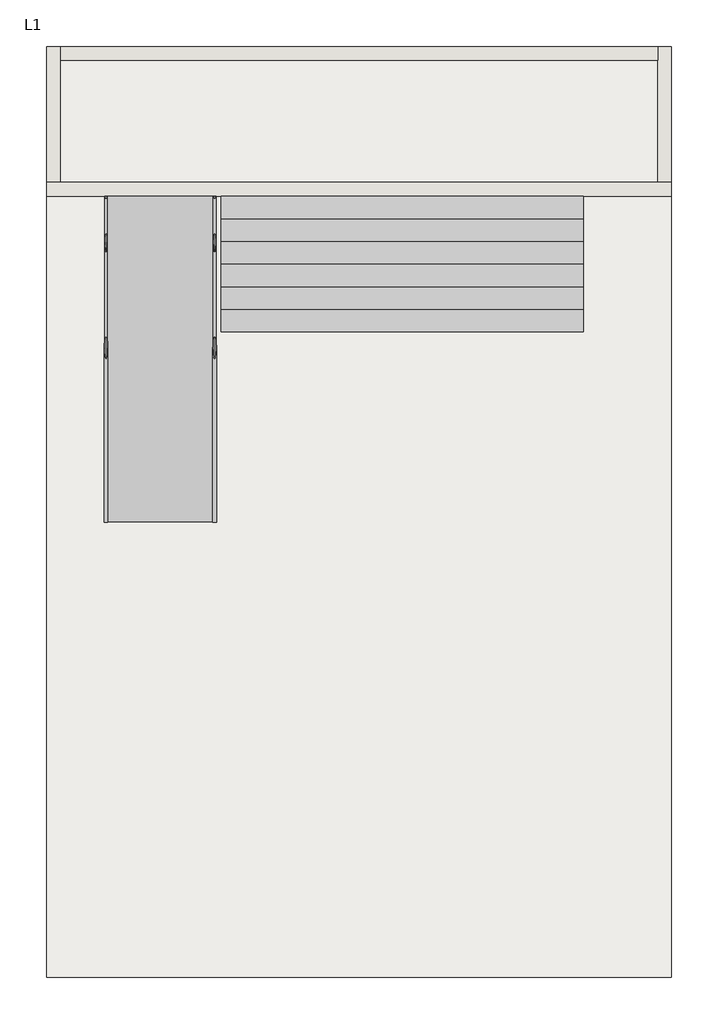
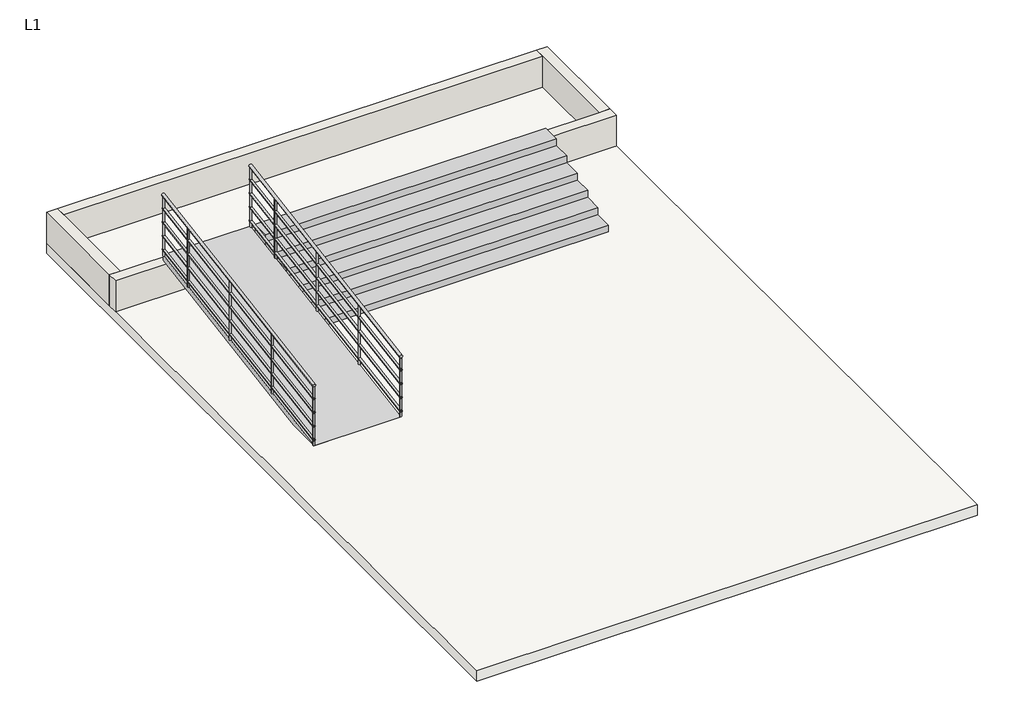
# One storey: 4 walls, 2 railings, 1 ramp, 1 slab, 1 stair flight.
"""IFC4 building model written with IfcOpenShell, lengths in millimetres."""

import ifcopenshell
import ifcopenshell.guid

model = None  # the IFC model being written
_history = None  # IfcOwnerHistory: only IFC2X3 demands one
_inside = {}  # id of a spatial element -> (the spatial element, [elements in it])
_under = {}  # id of a project, library or spatial element -> (it, [spatial elements below it])
_declared = {}  # id of a project -> (the project, [libraries it declares])
_typed = {}  # id of a type object -> (the type object, [elements of that type])
_made_of = {}  # id of a material, layer set ... -> (it, [elements and type objects made of it])


def new_model(schema):
    """Start an empty IFC model of exactly this schema.

    Asked for "IFC4X3", IfcOpenShell would pick the latest addendum, in which some entities
    have other attributes; the version numbers below select the first issue.
    IFC2X3 requires an IfcOwnerHistory on every rooted entity: one is made here for all.
    """
    global model, _history
    if schema == "IFC4X3":
        model = ifcopenshell.file(schema_version=(4, 3, 0, 0))
    else:
        model = ifcopenshell.file(schema=schema)
    _inside.clear()
    _under.clear()
    _declared.clear()
    _typed.clear()
    _made_of.clear()
    _history = None
    if model.schema == "IFC2X3":
        org = make("IfcOrganization", Name="unknown")
        user = make(
            "IfcPersonAndOrganization",
            ThePerson=make("IfcPerson", FamilyName="unknown"),
            TheOrganization=org,
        )
        app = make(
            "IfcApplication",
            ApplicationDeveloper=org,
            Version="unknown",
            ApplicationFullName="unknown",
            ApplicationIdentifier="unknown",
        )
        _history = make(
            "IfcOwnerHistory",
            OwningUser=user,
            OwningApplication=app,
            ChangeAction="ADDED",
            CreationDate=0,
        )
    return model


def make(cls, **values):
    """One entity of the class cls with the attributes given. An attribute that is None is left unset."""
    return model.create_entity(
        cls, **{name: value for name, value in values.items() if value is not None}
    )


def rooted(cls, **values):
    """An entity with a GlobalId (a new one), such as an element, a storey or a relation."""
    return make(cls, GlobalId=ifcopenshell.guid.new(), OwnerHistory=_history, **values)


def si_unit(unit_type, name, prefix=None):
    """IfcSIUnit, for example si_unit("LENGTHUNIT", "METRE", prefix="MILLI")."""
    return make("IfcSIUnit", UnitType=unit_type, Prefix=prefix, Name=name)


def assignment(units):
    """IfcUnitAssignment: the units of a project."""
    return None if units is None else make("IfcUnitAssignment", Units=units)


def point(xyz):
    """IfcCartesianPoint."""
    return None if xyz is None else make("IfcCartesianPoint", Coordinates=xyz)


def direction(xyz):
    """IfcDirection."""
    return None if xyz is None else make("IfcDirection", DirectionRatios=xyz)


def frame(location, z_axis=None, x_axis=None):
    """IfcAxis2Placement3D, a coordinate frame: its origin and axes. An axis left out is left unset."""
    return make(
        "IfcAxis2Placement3D",
        Location=point(location),
        Axis=direction(z_axis),
        RefDirection=direction(x_axis),
    )


def origin():
    """The frame at (0, 0, 0) with its axes left unset."""
    return frame((0.0, 0.0, 0.0))


def origin_with_axes():
    """The frame at (0, 0, 0) with the z axis (0, 0, 1) and the x axis (1, 0, 0) written out."""
    return frame((0.0, 0.0, 0.0), z_axis=(0.0, 0.0, 1.0), x_axis=(1.0, 0.0, 0.0))


def place(relative_to, where):
    """IfcLocalPlacement: puts the frame where relative to a parent placement (None: the world)."""
    return make(
        "IfcLocalPlacement", PlacementRelTo=relative_to, RelativePlacement=where
    )


def context(
    kind, dimensions, precision=None, world=None, true_north=None, identifier=None
):
    """IfcGeometricRepresentationContext, for example the 3D "Model" context."""
    return make(
        "IfcGeometricRepresentationContext",
        ContextIdentifier=identifier,
        ContextType=kind,
        CoordinateSpaceDimension=dimensions,
        Precision=precision,
        WorldCoordinateSystem=world,
        TrueNorth=true_north,
    )


def project(units=None, contexts=None):
    """IfcProject with its units and contexts."""
    return rooted(
        "IfcProject",
        Name="project",
        RepresentationContexts=contexts,
        UnitsInContext=assignment(units),
    )


def spatial(cls, under=None, at=None, **own):
    """A site, building, storey or space (cls), placed at a placement, below another one or the project."""
    s = rooted(cls, ObjectPlacement=at, **own)
    if under is not None:
        _under.setdefault(under.id(), (under, []))[1].append(s)
    return s


def polyline(points):
    """IfcPolyline through the points."""
    return make("IfcPolyline", Points=[point(p) for p in points])


def ellipse_curve(where, semi_axis1, semi_axis2):
    """IfcEllipse in the frame where."""
    return make(
        "IfcEllipse", Position=where, SemiAxis1=semi_axis1, SemiAxis2=semi_axis2
    )


def outline(outer, holes=None, kind="AREA"):
    """IfcArbitraryClosedProfileDef: a profile drawn as a closed curve; with holes, ...WithVoids."""
    if holes is None:
        return make("IfcArbitraryClosedProfileDef", ProfileType=kind, OuterCurve=outer)
    return make(
        "IfcArbitraryProfileDefWithVoids",
        ProfileType=kind,
        OuterCurve=outer,
        InnerCurves=holes,
    )


def extrude(swept, where, along, depth):
    """IfcExtrudedAreaSolid: the profile swept, set in the frame where, extruded along a direction by depth."""
    return make(
        "IfcExtrudedAreaSolid",
        SweptArea=swept,
        Position=where,
        ExtrudedDirection=direction(along),
        Depth=depth,
    )


def faces_of(points, faces, orient=None, outer=None):
    """IfcFace entities. A face is a list of loops; a loop is a list of indices into points, from 0.

    orient and outer hold one flag for each loop. By default every Orientation is true, the
    first loop of a face is its IfcFaceOuterBound and the others are IfcFaceBound.
    """
    made = []
    for i, loops in enumerate(faces):
        bounds = []
        for j, loop in enumerate(loops):
            is_outer = j == 0 if outer is None else outer[i][j]
            bounds.append(
                make(
                    "IfcFaceOuterBound" if is_outer else "IfcFaceBound",
                    Bound=make("IfcPolyLoop", Polygon=[points[k] for k in loop]),
                    Orientation=True if orient is None else orient[i][j],
                )
            )
        made.append(make("IfcFace", Bounds=bounds))
    return made


def faceted_brep(points, faces, orient=None, outer=None, voids=None):
    """IfcFacetedBrep: a solid bounded by flat faces; with voids (closed shells), ...WithVoids."""
    shared = [point(p) for p in points]
    hull = make("IfcClosedShell", CfsFaces=faces_of(shared, faces, orient, outer))
    if voids is None:
        return make("IfcFacetedBrep", Outer=hull)
    return make(
        "IfcFacetedBrepWithVoids",
        Outer=hull,
        Voids=[
            make(cls, CfsFaces=faces_of(shared, fs, o, b)) for cls, fs, o, b in voids
        ],
    )


def shape(context_of_items, identifier, shape_type, items):
    """IfcShapeRepresentation: the items that make up one representation, for example the "Body"."""
    return make(
        "IfcShapeRepresentation",
        ContextOfItems=context_of_items,
        RepresentationIdentifier=identifier,
        RepresentationType=shape_type,
        Items=items,
    )


def source(mapping_origin, context_of_items, identifier, shape_type, items):
    """IfcRepresentationMap: a shape defined once, which mapped items show again and again."""
    return make(
        "IfcRepresentationMap",
        MappingOrigin=mapping_origin,
        MappedRepresentation=shape(context_of_items, identifier, shape_type, items),
    )


def transform(
    local_origin,
    x_axis=None,
    y_axis=None,
    z_axis=None,
    scale=None,
    scale2=None,
    scale3=None,
    uniform=True,
):
    """IfcCartesianTransformationOperator3D, or its non-uniform kind. x_axis, y_axis, z_axis: its Axis1, 2, 3."""
    if uniform:
        return make(
            "IfcCartesianTransformationOperator3D",
            Axis1=direction(x_axis),
            Axis2=direction(y_axis),
            LocalOrigin=point(local_origin),
            Scale=scale,
            Axis3=direction(z_axis),
        )
    return make(
        "IfcCartesianTransformationOperator3DnonUniform",
        Axis1=direction(x_axis),
        Axis2=direction(y_axis),
        LocalOrigin=point(local_origin),
        Scale=scale,
        Axis3=direction(z_axis),
        Scale2=scale2,
        Scale3=scale3,
    )


def mapped(mapping_source, mapping_target):
    """IfcMappedItem: shows the shape of a source again, moved by a transform."""
    return make(
        "IfcMappedItem", MappingSource=mapping_source, MappingTarget=mapping_target
    )


def made_of(thing, what):
    """Note that an element or type object is made of a material, layer set ...; save() writes the relation."""
    if what is not None:
        _made_of.setdefault(what.id(), (what, []))[1].append(thing)
    return thing


def element(
    cls,
    number,
    at=None,
    inside=None,
    cuts=None,
    type_object=None,
    material=None,
    context=None,
    identifier="Body",
    shape_type=None,
    held_by="IfcProductDefinitionShape",
    body=None,
    shapes=None,
    **own,
):
    """One element of the class cls, such as IfcWall. Its Tag is "e" and its number.

    at: its placement. inside: the storey or other place that contains it. cuts: it is an
    opening in that element (IfcRelVoidsElement). A single representation is given by context,
    identifier, shape_type and body (its items); several are given by shapes. held_by: the class
    of the entity that holds the representations. save() writes the other relations.
    """
    e = rooted(cls, Tag="e%d" % number, ObjectPlacement=at, **own)
    if body is not None:
        shapes = [shape(context, identifier, shape_type, body)]
    if shapes is not None:
        e.Representation = make(held_by, Representations=shapes)
    if inside is not None:
        _inside.setdefault(inside.id(), (inside, []))[1].append(e)
    if cuts is not None:
        rooted(
            "IfcRelVoidsElement", RelatingBuildingElement=cuts, RelatedOpeningElement=e
        )
    if type_object is not None:
        _typed.setdefault(type_object.id(), (type_object, []))[1].append(e)
    return made_of(e, material)


def aggregate(whole, parts):
    """IfcRelAggregates: a whole, such as a stair, and the parts it consists of."""
    return rooted("IfcRelAggregates", RelatingObject=whole, RelatedObjects=parts)


def save(model, path):
    """Write the relations noted so far, then the file.

    IfcRelAggregates (storeys below a building ...), IfcRelContainedInSpatialStructure (elements
    in a storey), IfcRelDefinesByType, IfcRelAssociatesMaterial and IfcRelDeclares: one each for
    every whole, place, type object, material and project.
    """
    for whole, parts in _under.values():
        aggregate(whole, parts)
    for where, things in _inside.values():
        rooted(
            "IfcRelContainedInSpatialStructure",
            RelatedElements=things,
            RelatingStructure=where,
        )
    for kind, things in _typed.values():
        rooted("IfcRelDefinesByType", RelatedObjects=things, RelatingType=kind)
    for what, things in _made_of.values():
        rooted("IfcRelAssociatesMaterial", RelatedObjects=things, RelatingMaterial=what)
    for by, libraries in _declared.values():
        rooted("IfcRelDeclares", RelatingContext=by, RelatedDefinitions=libraries)
    model.write(path)


def plane_surface(at):
    """IfcPlane: the flat surface through the origin of the frame at, square to its z axis."""
    return make("IfcPlane", Position=at)


def cylinder_surface(at, radius):
    """IfcCylindricalSurface: all points at the distance radius from the z axis of the frame at."""
    return make("IfcCylindricalSurface", Position=at, Radius=radius)


def advanced_brep(points, edges, surfaces, faces):
    """IfcAdvancedBrep: a solid bounded by faces that lie on surfaces and meet in shared edges.

    An edge is (start, end): straight between two places in points (the first is 0);
    or (start, end, curve); or (start, end, curve, False) where it runs against its curve.
    A face is (place in surfaces, loops), or (place, loops, False) where it looks against
    its surface's normal. A loop lists edges by number (the first is 1), with a minus sign
    where the edge is run from its end to its start. The first loop is the outer one.
    """
    corners = [point(p) for p in points]
    vertices = [make("IfcVertexPoint", VertexGeometry=c) for c in corners]
    made = []
    for start, end, *more in edges:
        made.append(
            make(
                "IfcEdgeCurve",
                EdgeStart=vertices[start],
                EdgeEnd=vertices[end],
                EdgeGeometry=more[0] if more else make("IfcPolyline", Points=[corners[start], corners[end]]),
                SameSense=more[1] if len(more) > 1 else True,
            )
        )
    hull = []
    for where, loops, *sense in faces:
        bounds = []
        for j, loop in enumerate(loops):
            ring = [make("IfcOrientedEdge", EdgeElement=made[abs(k) - 1], Orientation=k > 0) for k in loop]
            bounds.append(
                make(
                    "IfcFaceOuterBound" if j == 0 else "IfcFaceBound",
                    Bound=make("IfcEdgeLoop", EdgeList=ring),
                    Orientation=True,
                )
            )
        hull.append(make("IfcAdvancedFace", Bounds=bounds, FaceSurface=surfaces[where], SameSense=sense[0] if sense else True))
    return make("IfcAdvancedBrep", Outer=make("IfcClosedShell", CfsFaces=hull))


def ramp_1_7f35b39e(model_context):
    return source(origin(), model_context, "Body", "SweptSolid", [
        extrude(outline(polyline([(-4458.4292912, 0.0), (-858.4292912, 600.0), (-858.4292912, 523.9654684), (-4458.4292912, -76.0345316), (-4458.4292912, 0.0)])), frame((-599.8488078, 0.0, 0.0), z_axis=(1.0, 0.0, 0.0), x_axis=(0.0, 1.0, 0.0)), (0.0, 0.0, 1.0), 1200.0),
    ])


model = new_model("IFC4")

# Units and contexts
model_context = context("Model", 3, world=origin())
ifc_project = project(units=[si_unit("LENGTHUNIT", "METRE", prefix="MILLI")], contexts=[model_context])

# Site, building, storey
site = spatial("IfcSite", under=ifc_project)
building = spatial("IfcBuilding", under=site)
storey = spatial("IfcBuildingStorey", under=building, Name="L1", Elevation=0.0)

# Railings
placement = place(None, origin())
element("IfcRailing", 1, ObjectType="900mm Pipe", at=placement, inside=storey, context=model_context, shape_type="AdvancedBrep", body=[
    advanced_brep(
    [(620.1511922, -4458.4292912, 879.7241249), (580.1511922, -4458.4292912, 879.7241249), (620.1511922, -858.4292912, 1479.7241249), (580.1511922, -858.4292912, 1479.7241249)],
    [
        (0, 1, ellipse_curve(frame((600.1511922, -4458.4292912, 879.7241249), z_axis=(0.0, -1.0, 0.0), x_axis=(0.0, 0.0, -1.0)), 20.2758751, 20.0)),
        (1, 0, ellipse_curve(frame((600.1511922, -4458.4292912, 879.7241249), z_axis=(0.0, -1.0, 0.0), x_axis=(0.0, 0.0, -1.0)), 20.2758751, 20.0)),
        (2, 3, ellipse_curve(frame((600.1511922, -858.4292912, 1479.7241249), z_axis=(0.0, 1.0, 0.0), x_axis=(0.0, 0.0, -1.0)), 20.2758751, 20.0)),
        (3, 2, ellipse_curve(frame((600.1511922, -858.4292912, 1479.7241249), z_axis=(0.0, 1.0, 0.0), x_axis=(0.0, 0.0, -1.0)), 20.2758751, 20.0)),
        (0, 2),
        (3, 1),
    ],
    [
        plane_surface(frame((600.1511922, -4458.4292912, 900.0), z_axis=(0.0, -1.0, 0.0), x_axis=(0.0, 0.0, 1.0))),
        plane_surface(frame((600.1511922, -858.4292912, 1500.0), z_axis=(0.0, 1.0, 0.0), x_axis=(0.0, 0.0, 1.0))),
        cylinder_surface(frame((600.1511922, -4455.1413114, 880.2721215), z_axis=(0.0, -0.9863939238321437, -0.16439898730535737), x_axis=(-1.0, 0.0, 0.0)), 20.0),
    ],
    [
        (0, [[1, 2]]),
        (1, [[3, 4]]),
        (2, [[-1, 5, -4, 6]]),
        (2, [[-2, -6, -3, -5]]),
    ],
),
    advanced_brep(
    [(615.1511922, -4458.4292912, 684.7930937), (585.1511922, -4458.4292912, 684.7930937), (615.1511922, -858.4292912, 1284.7930937), (585.1511922, -858.4292912, 1284.7930937)],
    [
        (0, 1, ellipse_curve(frame((600.1511922, -4458.4292912, 684.7930937), z_axis=(0.0, -1.0, 0.0), x_axis=(0.0, 0.0, -1.0)), 15.2069063, 15.0)),
        (1, 0, ellipse_curve(frame((600.1511922, -4458.4292912, 684.7930937), z_axis=(0.0, -1.0, 0.0), x_axis=(0.0, 0.0, -1.0)), 15.2069063, 15.0)),
        (2, 3, ellipse_curve(frame((600.1511922, -858.4292912, 1284.7930937), z_axis=(0.0, 1.0, 0.0), x_axis=(0.0, 0.0, -1.0)), 15.2069063, 15.0)),
        (3, 2, ellipse_curve(frame((600.1511922, -858.4292912, 1284.7930937), z_axis=(0.0, 1.0, 0.0), x_axis=(0.0, 0.0, -1.0)), 15.2069063, 15.0)),
        (0, 2),
        (3, 1),
    ],
    [
        plane_surface(frame((600.1511922, -4458.4292912, 700.0), z_axis=(0.0, -1.0, 0.0), x_axis=(0.0, 0.0, 1.0))),
        plane_surface(frame((600.1511922, -858.4292912, 1300.0), z_axis=(0.0, 1.0, 0.0), x_axis=(0.0, 0.0, 1.0))),
        cylinder_surface(frame((600.1511922, -4455.9633063, 685.2040911), z_axis=(0.0, -0.9863939238321437, -0.16439898730535732), x_axis=(-1.0, 0.0, 0.0)), 15.0),
    ],
    [
        (0, [[1, 2]]),
        (1, [[3, 4]]),
        (2, [[-1, 5, -4, 6]]),
        (2, [[-2, -6, -3, -5]]),
    ],
),
    advanced_brep(
    [(615.1511922, -4458.4292912, 484.7930937), (585.1511922, -4458.4292912, 484.7930937), (615.1511922, -858.4292912, 1084.7930937), (585.1511922, -858.4292912, 1084.7930937)],
    [
        (0, 1, ellipse_curve(frame((600.1511922, -4458.4292912, 484.7930937), z_axis=(0.0, -1.0, 0.0), x_axis=(0.0, 0.0, -1.0)), 15.2069063, 15.0)),
        (1, 0, ellipse_curve(frame((600.1511922, -4458.4292912, 484.7930937), z_axis=(0.0, -1.0, 0.0), x_axis=(0.0, 0.0, -1.0)), 15.2069063, 15.0)),
        (2, 3, ellipse_curve(frame((600.1511922, -858.4292912, 1084.7930937), z_axis=(0.0, 1.0, 0.0), x_axis=(0.0, 0.0, -1.0)), 15.2069063, 15.0)),
        (3, 2, ellipse_curve(frame((600.1511922, -858.4292912, 1084.7930937), z_axis=(0.0, 1.0, 0.0), x_axis=(0.0, 0.0, -1.0)), 15.2069063, 15.0)),
        (0, 2),
        (3, 1),
    ],
    [
        plane_surface(frame((600.1511922, -4458.4292912, 500.0), z_axis=(0.0, -1.0, 0.0), x_axis=(0.0, 0.0, 1.0))),
        plane_surface(frame((600.1511922, -858.4292912, 1100.0), z_axis=(0.0, 1.0, 0.0), x_axis=(0.0, 0.0, 1.0))),
        cylinder_surface(frame((600.1511922, -4455.9633063, 485.2040911), z_axis=(0.0, -0.9863939238321437, -0.16439898730535732), x_axis=(-1.0, 0.0, 0.0)), 15.0),
    ],
    [
        (0, [[1, 2]]),
        (1, [[3, 4]]),
        (2, [[-1, 5, -4, 6]]),
        (2, [[-2, -6, -3, -5]]),
    ],
),
    advanced_brep(
    [(615.1511922, -4458.4292912, 284.7930937), (585.1511922, -4458.4292912, 284.7930937), (615.1511922, -858.4292912, 884.7930937), (585.1511922, -858.4292912, 884.7930937)],
    [
        (0, 1, ellipse_curve(frame((600.1511922, -4458.4292912, 284.7930937), z_axis=(0.0, -1.0, 0.0), x_axis=(0.0, 0.0, -1.0)), 15.2069063, 15.0)),
        (1, 0, ellipse_curve(frame((600.1511922, -4458.4292912, 284.7930937), z_axis=(0.0, -1.0, 0.0), x_axis=(0.0, 0.0, -1.0)), 15.2069063, 15.0)),
        (2, 3, ellipse_curve(frame((600.1511922, -858.4292912, 884.7930937), z_axis=(0.0, 1.0, 0.0), x_axis=(0.0, 0.0, -1.0)), 15.2069063, 15.0)),
        (3, 2, ellipse_curve(frame((600.1511922, -858.4292912, 884.7930937), z_axis=(0.0, 1.0, 0.0), x_axis=(0.0, 0.0, -1.0)), 15.2069063, 15.0)),
        (0, 2),
        (3, 1),
    ],
    [
        plane_surface(frame((600.1511922, -4458.4292912, 300.0), z_axis=(0.0, -1.0, 0.0), x_axis=(0.0, 0.0, 1.0))),
        plane_surface(frame((600.1511922, -858.4292912, 900.0), z_axis=(0.0, 1.0, 0.0), x_axis=(0.0, 0.0, 1.0))),
        cylinder_surface(frame((600.1511922, -4455.9633063, 285.2040911), z_axis=(0.0, -0.9863939238321437, -0.16439898730535732), x_axis=(-1.0, 0.0, 0.0)), 15.0),
    ],
    [
        (0, [[1, 2]]),
        (1, [[3, 4]]),
        (2, [[-1, 5, -4, 6]]),
        (2, [[-2, -6, -3, -5]]),
    ],
),
    advanced_brep(
    [(615.1511922, -4458.4292912, 84.7930937), (585.1511922, -4458.4292912, 84.7930937), (615.1511922, -858.4292912, 684.7930937), (585.1511922, -858.4292912, 684.7930937)],
    [
        (0, 1, ellipse_curve(frame((600.1511922, -4458.4292912, 84.7930937), z_axis=(0.0, -1.0, 0.0), x_axis=(0.0, 0.0, -1.0)), 15.2069063, 15.0)),
        (1, 0, ellipse_curve(frame((600.1511922, -4458.4292912, 84.7930937), z_axis=(0.0, -1.0, 0.0), x_axis=(0.0, 0.0, -1.0)), 15.2069063, 15.0)),
        (2, 3, ellipse_curve(frame((600.1511922, -858.4292912, 684.7930937), z_axis=(0.0, 1.0, 0.0), x_axis=(0.0, 0.0, -1.0)), 15.2069063, 15.0)),
        (3, 2, ellipse_curve(frame((600.1511922, -858.4292912, 684.7930937), z_axis=(0.0, 1.0, 0.0), x_axis=(0.0, 0.0, -1.0)), 15.2069063, 15.0)),
        (0, 2),
        (3, 1),
    ],
    [
        plane_surface(frame((600.1511922, -4458.4292912, 100.0), z_axis=(0.0, -1.0, 0.0), x_axis=(0.0, 0.0, 1.0))),
        plane_surface(frame((600.1511922, -858.4292912, 700.0), z_axis=(0.0, 1.0, 0.0), x_axis=(0.0, 0.0, 1.0))),
        cylinder_surface(frame((600.1511922, -4455.9633063, 85.2040911), z_axis=(0.0, -0.9863939238321437, -0.16439898730535732), x_axis=(-1.0, 0.0, 0.0)), 15.0),
    ],
    [
        (0, [[1, 2]]),
        (1, [[3, 4]]),
        (2, [[-1, 5, -4, 6]]),
        (2, [[-2, -6, -3, -5]]),
    ],
),
    advanced_brep(
    [(587.6511922, -1458.4292912, 1359.4482498), (612.6511922, -1458.4292912, 1359.4482498), (612.6511922, -1458.4292912, 500.0), (587.6511922, -1458.4292912, 500.0)],
    [
        (0, 1, ellipse_curve(frame((600.1511922, -1458.4292912, 1359.4482498), z_axis=(0.0, 0.1643989873053573, -0.9863939238321439), x_axis=(0.0, 0.9863939238321439, 0.1643989873053556)), 12.6724219, 12.5)),
        (1, 2),
        (2, 3, ellipse_curve(frame((600.1511922, -1458.4292912, 500.0), z_axis=(0.0, -0.16439898730535726, 0.9863939238321439), x_axis=(0.0, 0.9863939238321439, 0.16439898730535563)), 12.6724219, 12.5)),
        (3, 0),
        (3, 2, ellipse_curve(frame((600.1511922, -1458.4292912, 500.0), z_axis=(0.0, -0.16439898730535726, 0.9863939238321439), x_axis=(0.0, 0.9863939238321439, 0.16439898730535563)), 12.6724219, 12.5)),
        (1, 0, ellipse_curve(frame((600.1511922, -1458.4292912, 1359.4482498), z_axis=(0.0, 0.1643989873053573, -0.9863939238321439), x_axis=(0.0, 0.9863939238321439, 0.1643989873053556)), 12.6724219, 12.5)),
    ],
    [
        cylinder_surface(frame((600.1511922, -1458.4292912, 400.0), z_axis=(0.0, 0.0, 1.0), x_axis=(1.0, 0.0, 0.0)), 12.5),
        plane_surface(frame((625.1511922, -1433.4292912, 1363.6149165), z_axis=(0.0, -0.1643989873053573, 0.9863939238321439), x_axis=(-1.0, 0.0, 0.0))),
        plane_surface(frame((625.1511922, -1483.4292912, 495.8333333), z_axis=(0.0, 0.16439898730535726, -0.9863939238321439), x_axis=(-1.0, 0.0, 0.0))),
    ],
    [
        (0, [[1, 2, 3, 4]]),
        (0, [[5, -2, 6, -4]]),
        (1, [[-6, -1]]),
        (2, [[-5, -3]]),
    ],
),
    advanced_brep(
    [(587.6511922, -2458.4292912, 1192.7815831), (612.6511922, -2458.4292912, 1192.7815831), (612.6511922, -2458.4292912, 333.3333333), (587.6511922, -2458.4292912, 333.3333333)],
    [
        (0, 1, ellipse_curve(frame((600.1511922, -2458.4292912, 1192.7815831), z_axis=(0.0, 0.1643989873053573, -0.9863939238321439), x_axis=(0.0, 0.9863939238321439, 0.1643989873053556)), 12.6724219, 12.5)),
        (1, 2),
        (2, 3, ellipse_curve(frame((600.1511922, -2458.4292912, 333.3333333), z_axis=(0.0, -0.16439898730535726, 0.9863939238321439), x_axis=(0.0, 0.9863939238321439, 0.16439898730535563)), 12.6724219, 12.5)),
        (3, 0),
        (3, 2, ellipse_curve(frame((600.1511922, -2458.4292912, 333.3333333), z_axis=(0.0, -0.16439898730535726, 0.9863939238321439), x_axis=(0.0, 0.9863939238321439, 0.16439898730535563)), 12.6724219, 12.5)),
        (1, 0, ellipse_curve(frame((600.1511922, -2458.4292912, 1192.7815831), z_axis=(0.0, 0.1643989873053573, -0.9863939238321439), x_axis=(0.0, 0.9863939238321439, 0.1643989873053556)), 12.6724219, 12.5)),
    ],
    [
        cylinder_surface(frame((600.1511922, -2458.4292912, 233.3333333), z_axis=(0.0, 0.0, 1.0), x_axis=(1.0, 0.0, 0.0)), 12.5),
        plane_surface(frame((625.1511922, -2433.4292912, 1196.9482498), z_axis=(0.0, -0.1643989873053573, 0.9863939238321439), x_axis=(-1.0, 0.0, 0.0))),
        plane_surface(frame((625.1511922, -2483.4292912, 329.1666667), z_axis=(0.0, 0.16439898730535726, -0.9863939238321439), x_axis=(-1.0, 0.0, 0.0))),
    ],
    [
        (0, [[1, 2, 3, 4]]),
        (0, [[5, -2, 6, -4]]),
        (1, [[-6, -1]]),
        (2, [[-5, -3]]),
    ],
),
    advanced_brep(
    [(587.6511922, -3458.4292912, 1026.1149165), (612.6511922, -3458.4292912, 1026.1149165), (612.6511922, -3458.4292912, 166.6666667), (587.6511922, -3458.4292912, 166.6666667)],
    [
        (0, 1, ellipse_curve(frame((600.1511922, -3458.4292912, 1026.1149165), z_axis=(0.0, 0.1643989873053573, -0.9863939238321439), x_axis=(0.0, 0.9863939238321439, 0.1643989873053556)), 12.6724219, 12.5)),
        (1, 2),
        (2, 3, ellipse_curve(frame((600.1511922, -3458.4292912, 166.6666667), z_axis=(0.0, -0.16439898730535726, 0.9863939238321439), x_axis=(0.0, 0.9863939238321439, 0.16439898730535563)), 12.6724219, 12.5)),
        (3, 0),
        (3, 2, ellipse_curve(frame((600.1511922, -3458.4292912, 166.6666667), z_axis=(0.0, -0.16439898730535726, 0.9863939238321439), x_axis=(0.0, 0.9863939238321439, 0.16439898730535563)), 12.6724219, 12.5)),
        (1, 0, ellipse_curve(frame((600.1511922, -3458.4292912, 1026.1149165), z_axis=(0.0, 0.1643989873053573, -0.9863939238321439), x_axis=(0.0, 0.9863939238321439, 0.1643989873053556)), 12.6724219, 12.5)),
    ],
    [
        cylinder_surface(frame((600.1511922, -3458.4292912, 66.6666667), z_axis=(0.0, 0.0, 1.0), x_axis=(1.0, 0.0, 0.0)), 12.5),
        plane_surface(frame((625.1511922, -3433.4292912, 1030.2815831), z_axis=(0.0, -0.1643989873053573, 0.9863939238321439), x_axis=(-1.0, 0.0, 0.0))),
        plane_surface(frame((625.1511922, -3483.4292912, 162.5), z_axis=(0.0, 0.16439898730535726, -0.9863939238321439), x_axis=(-1.0, 0.0, 0.0))),
    ],
    [
        (0, [[1, 2, 3, 4]]),
        (0, [[5, -2, 6, -4]]),
        (1, [[-6, -1]]),
        (2, [[-5, -3]]),
    ],
),
    advanced_brep(
    [(587.6511922, -870.9292912, 1457.3649165), (612.6511922, -870.9292912, 1457.3649165), (612.6511922, -870.9292912, 597.9166667), (587.6511922, -870.9292912, 597.9166667)],
    [
        (0, 1, ellipse_curve(frame((600.1511922, -870.9292912, 1457.3649165), z_axis=(0.0, 0.1643989873053573, -0.9863939238321439), x_axis=(0.0, 0.9863939238321439, 0.1643989873053556)), 12.6724219, 12.5)),
        (1, 2),
        (2, 3, ellipse_curve(frame((600.1511922, -870.9292912, 597.9166667), z_axis=(0.0, -0.16439898730535726, 0.9863939238321439), x_axis=(0.0, 0.9863939238321439, 0.16439898730535563)), 12.6724219, 12.5)),
        (3, 0),
        (3, 2, ellipse_curve(frame((600.1511922, -870.9292912, 597.9166667), z_axis=(0.0, -0.16439898730535726, 0.9863939238321439), x_axis=(0.0, 0.9863939238321439, 0.16439898730535563)), 12.6724219, 12.5)),
        (1, 0, ellipse_curve(frame((600.1511922, -870.9292912, 1457.3649165), z_axis=(0.0, 0.1643989873053573, -0.9863939238321439), x_axis=(0.0, 0.9863939238321439, 0.1643989873053556)), 12.6724219, 12.5)),
    ],
    [
        cylinder_surface(frame((600.1511922, -870.9292912, 497.9166667), z_axis=(0.0, 0.0, 1.0), x_axis=(1.0, 0.0, 0.0)), 12.5),
        plane_surface(frame((625.1511922, -845.9292912, 1461.5315831), z_axis=(0.0, -0.1643989873053573, 0.9863939238321439), x_axis=(-1.0, 0.0, 0.0))),
        plane_surface(frame((625.1511922, -895.9292912, 593.75), z_axis=(0.0, 0.16439898730535726, -0.9863939238321439), x_axis=(-1.0, 0.0, 0.0))),
    ],
    [
        (0, [[1, 2, 3, 4]]),
        (0, [[5, -2, 6, -4]]),
        (1, [[-6, -1]]),
        (2, [[-5, -3]]),
    ],
),
    advanced_brep(
    [(587.6511922, -4445.9292912, 861.5315831), (612.6511922, -4445.9292912, 861.5315831), (612.6511922, -4445.9292912, 2.0833333), (587.6511922, -4445.9292912, 2.0833333)],
    [
        (0, 1, ellipse_curve(frame((600.1511922, -4445.9292912, 861.5315831), z_axis=(0.0, 0.1643989873053573, -0.9863939238321439), x_axis=(0.0, 0.9863939238321439, 0.1643989873053556)), 12.6724219, 12.5)),
        (1, 2),
        (2, 3, ellipse_curve(frame((600.1511922, -4445.9292912, 2.0833333), z_axis=(0.0, -0.16439898730535726, 0.9863939238321439), x_axis=(0.0, 0.9863939238321439, 0.16439898730535563)), 12.6724219, 12.5)),
        (3, 0),
        (3, 2, ellipse_curve(frame((600.1511922, -4445.9292912, 2.0833333), z_axis=(0.0, -0.16439898730535726, 0.9863939238321439), x_axis=(0.0, 0.9863939238321439, 0.16439898730535563)), 12.6724219, 12.5)),
        (1, 0, ellipse_curve(frame((600.1511922, -4445.9292912, 861.5315831), z_axis=(0.0, 0.1643989873053573, -0.9863939238321439), x_axis=(0.0, 0.9863939238321439, 0.1643989873053556)), 12.6724219, 12.5)),
    ],
    [
        cylinder_surface(frame((600.1511922, -4445.9292912, -97.9166667), z_axis=(0.0, 0.0, 1.0), x_axis=(1.0, 0.0, 0.0)), 12.5),
        plane_surface(frame((625.1511922, -4420.9292912, 865.6982498), z_axis=(0.0, -0.1643989873053573, 0.9863939238321439), x_axis=(-1.0, 0.0, 0.0))),
        plane_surface(frame((625.1511922, -4470.9292912, -2.0833333), z_axis=(0.0, 0.16439898730535726, -0.9863939238321439), x_axis=(-1.0, 0.0, 0.0))),
    ],
    [
        (0, [[1, 2, 3, 4]]),
        (0, [[5, -2, 6, -4]]),
        (1, [[-6, -1]]),
        (2, [[-5, -3]]),
    ],
),
])
element("IfcRailing", 2, ObjectType="900mm Pipe", at=placement, inside=storey, context=model_context, shape_type="AdvancedBrep", body=[
    advanced_brep(
    [(-579.8488078, -4458.4292912, 879.7241249), (-619.8488078, -4458.4292912, 879.7241249), (-579.8488078, -858.4292912, 1479.7241249), (-619.8488078, -858.4292912, 1479.7241249)],
    [
        (0, 1, ellipse_curve(frame((-599.8488078, -4458.4292912, 879.7241249), z_axis=(0.0, -1.0, 0.0), x_axis=(0.0, 0.0, -1.0)), 20.2758751, 20.0)),
        (1, 0, ellipse_curve(frame((-599.8488078, -4458.4292912, 879.7241249), z_axis=(0.0, -1.0, 0.0), x_axis=(0.0, 0.0, -1.0)), 20.2758751, 20.0)),
        (2, 3, ellipse_curve(frame((-599.8488078, -858.4292912, 1479.7241249), z_axis=(0.0, 1.0, 0.0), x_axis=(0.0, 0.0, -1.0)), 20.2758751, 20.0)),
        (3, 2, ellipse_curve(frame((-599.8488078, -858.4292912, 1479.7241249), z_axis=(0.0, 1.0, 0.0), x_axis=(0.0, 0.0, -1.0)), 20.2758751, 20.0)),
        (0, 2),
        (3, 1),
    ],
    [
        plane_surface(frame((-599.8488078, -4458.4292912, 900.0), z_axis=(0.0, -1.0, 0.0), x_axis=(0.0, 0.0, 1.0))),
        plane_surface(frame((-599.8488078, -858.4292912, 1500.0), z_axis=(0.0, 1.0, 0.0), x_axis=(0.0, 0.0, 1.0))),
        cylinder_surface(frame((-599.8488078, -4455.1413114, 880.2721215), z_axis=(0.0, -0.9863939238321437, -0.16439898730535737), x_axis=(-1.0, 0.0, 0.0)), 20.0),
    ],
    [
        (0, [[1, 2]]),
        (1, [[3, 4]]),
        (2, [[-1, 5, -4, 6]]),
        (2, [[-2, -6, -3, -5]]),
    ],
),
    advanced_brep(
    [(-614.8488078, -4458.4292912, 684.7930937), (-584.8488078, -4458.4292912, 684.7930937), (-614.8488078, -858.4292912, 1284.7930937), (-584.8488078, -858.4292912, 1284.7930937)],
    [
        (0, 1, ellipse_curve(frame((-599.8488078, -4458.4292912, 684.7930937), z_axis=(0.0, -1.0, 0.0), x_axis=(0.0, 0.0, -1.0)), 15.2069063, 15.0)),
        (1, 0, ellipse_curve(frame((-599.8488078, -4458.4292912, 684.7930937), z_axis=(0.0, -1.0, 0.0), x_axis=(0.0, 0.0, -1.0)), 15.2069063, 15.0)),
        (2, 3, ellipse_curve(frame((-599.8488078, -858.4292912, 1284.7930937), z_axis=(0.0, 1.0, 0.0), x_axis=(0.0, 0.0, -1.0)), 15.2069063, 15.0)),
        (3, 2, ellipse_curve(frame((-599.8488078, -858.4292912, 1284.7930937), z_axis=(0.0, 1.0, 0.0), x_axis=(0.0, 0.0, -1.0)), 15.2069063, 15.0)),
        (0, 2),
        (3, 1),
    ],
    [
        plane_surface(frame((-599.8488078, -4458.4292912, 700.0), z_axis=(0.0, -1.0, 0.0), x_axis=(0.0, 0.0, 1.0))),
        plane_surface(frame((-599.8488078, -858.4292912, 1300.0), z_axis=(0.0, 1.0, 0.0), x_axis=(0.0, 0.0, 1.0))),
        cylinder_surface(frame((-599.8488078, -4455.9633063, 685.2040911), z_axis=(0.0, -0.9863939238321437, -0.16439898730535732), x_axis=(1.0, 0.0, 0.0)), 15.0),
    ],
    [
        (0, [[1, 2]]),
        (1, [[3, 4]]),
        (2, [[-1, 5, -4, 6]]),
        (2, [[-2, -6, -3, -5]]),
    ],
),
    advanced_brep(
    [(-614.8488078, -4458.4292912, 484.7930937), (-584.8488078, -4458.4292912, 484.7930937), (-614.8488078, -858.4292912, 1084.7930937), (-584.8488078, -858.4292912, 1084.7930937)],
    [
        (0, 1, ellipse_curve(frame((-599.8488078, -4458.4292912, 484.7930937), z_axis=(0.0, -1.0, 0.0), x_axis=(0.0, 0.0, -1.0)), 15.2069063, 15.0)),
        (1, 0, ellipse_curve(frame((-599.8488078, -4458.4292912, 484.7930937), z_axis=(0.0, -1.0, 0.0), x_axis=(0.0, 0.0, -1.0)), 15.2069063, 15.0)),
        (2, 3, ellipse_curve(frame((-599.8488078, -858.4292912, 1084.7930937), z_axis=(0.0, 1.0, 0.0), x_axis=(0.0, 0.0, -1.0)), 15.2069063, 15.0)),
        (3, 2, ellipse_curve(frame((-599.8488078, -858.4292912, 1084.7930937), z_axis=(0.0, 1.0, 0.0), x_axis=(0.0, 0.0, -1.0)), 15.2069063, 15.0)),
        (0, 2),
        (3, 1),
    ],
    [
        plane_surface(frame((-599.8488078, -4458.4292912, 500.0), z_axis=(0.0, -1.0, 0.0), x_axis=(0.0, 0.0, 1.0))),
        plane_surface(frame((-599.8488078, -858.4292912, 1100.0), z_axis=(0.0, 1.0, 0.0), x_axis=(0.0, 0.0, 1.0))),
        cylinder_surface(frame((-599.8488078, -4455.9633063, 485.2040911), z_axis=(0.0, -0.9863939238321437, -0.16439898730535732), x_axis=(1.0, 0.0, 0.0)), 15.0),
    ],
    [
        (0, [[1, 2]]),
        (1, [[3, 4]]),
        (2, [[-1, 5, -4, 6]]),
        (2, [[-2, -6, -3, -5]]),
    ],
),
    advanced_brep(
    [(-614.8488078, -4458.4292912, 284.7930937), (-584.8488078, -4458.4292912, 284.7930937), (-614.8488078, -858.4292912, 884.7930937), (-584.8488078, -858.4292912, 884.7930937)],
    [
        (0, 1, ellipse_curve(frame((-599.8488078, -4458.4292912, 284.7930937), z_axis=(0.0, -1.0, 0.0), x_axis=(0.0, 0.0, -1.0)), 15.2069063, 15.0)),
        (1, 0, ellipse_curve(frame((-599.8488078, -4458.4292912, 284.7930937), z_axis=(0.0, -1.0, 0.0), x_axis=(0.0, 0.0, -1.0)), 15.2069063, 15.0)),
        (2, 3, ellipse_curve(frame((-599.8488078, -858.4292912, 884.7930937), z_axis=(0.0, 1.0, 0.0), x_axis=(0.0, 0.0, -1.0)), 15.2069063, 15.0)),
        (3, 2, ellipse_curve(frame((-599.8488078, -858.4292912, 884.7930937), z_axis=(0.0, 1.0, 0.0), x_axis=(0.0, 0.0, -1.0)), 15.2069063, 15.0)),
        (0, 2),
        (3, 1),
    ],
    [
        plane_surface(frame((-599.8488078, -4458.4292912, 300.0), z_axis=(0.0, -1.0, 0.0), x_axis=(0.0, 0.0, 1.0))),
        plane_surface(frame((-599.8488078, -858.4292912, 900.0), z_axis=(0.0, 1.0, 0.0), x_axis=(0.0, 0.0, 1.0))),
        cylinder_surface(frame((-599.8488078, -4455.9633063, 285.2040911), z_axis=(0.0, -0.9863939238321437, -0.16439898730535732), x_axis=(1.0, 0.0, 0.0)), 15.0),
    ],
    [
        (0, [[1, 2]]),
        (1, [[3, 4]]),
        (2, [[-1, 5, -4, 6]]),
        (2, [[-2, -6, -3, -5]]),
    ],
),
    advanced_brep(
    [(-614.8488078, -4458.4292912, 84.7930937), (-584.8488078, -4458.4292912, 84.7930937), (-614.8488078, -858.4292912, 684.7930937), (-584.8488078, -858.4292912, 684.7930937)],
    [
        (0, 1, ellipse_curve(frame((-599.8488078, -4458.4292912, 84.7930937), z_axis=(0.0, -1.0, 0.0), x_axis=(0.0, 0.0, -1.0)), 15.2069063, 15.0)),
        (1, 0, ellipse_curve(frame((-599.8488078, -4458.4292912, 84.7930937), z_axis=(0.0, -1.0, 0.0), x_axis=(0.0, 0.0, -1.0)), 15.2069063, 15.0)),
        (2, 3, ellipse_curve(frame((-599.8488078, -858.4292912, 684.7930937), z_axis=(0.0, 1.0, 0.0), x_axis=(0.0, 0.0, -1.0)), 15.2069063, 15.0)),
        (3, 2, ellipse_curve(frame((-599.8488078, -858.4292912, 684.7930937), z_axis=(0.0, 1.0, 0.0), x_axis=(0.0, 0.0, -1.0)), 15.2069063, 15.0)),
        (0, 2),
        (3, 1),
    ],
    [
        plane_surface(frame((-599.8488078, -4458.4292912, 100.0), z_axis=(0.0, -1.0, 0.0), x_axis=(0.0, 0.0, 1.0))),
        plane_surface(frame((-599.8488078, -858.4292912, 700.0), z_axis=(0.0, 1.0, 0.0), x_axis=(0.0, 0.0, 1.0))),
        cylinder_surface(frame((-599.8488078, -4455.9633063, 85.2040911), z_axis=(0.0, -0.9863939238321437, -0.16439898730535732), x_axis=(1.0, 0.0, 0.0)), 15.0),
    ],
    [
        (0, [[1, 2]]),
        (1, [[3, 4]]),
        (2, [[-1, 5, -4, 6]]),
        (2, [[-2, -6, -3, -5]]),
    ],
),
    advanced_brep(
    [(-587.3488078, -1458.4292912, 1359.4482498), (-587.3488078, -1458.4292912, 500.0), (-612.3488078, -1458.4292912, 500.0), (-612.3488078, -1458.4292912, 1359.4482498)],
    [
        (0, 1),
        (1, 2, ellipse_curve(frame((-599.8488078, -1458.4292912, 500.0), z_axis=(0.0, -0.16439898730535726, 0.9863939238321439), x_axis=(0.0, 0.9863939238321439, 0.16439898730535563)), 12.6724219, 12.5)),
        (2, 3),
        (3, 0, ellipse_curve(frame((-599.8488078, -1458.4292912, 1359.4482498), z_axis=(0.0, 0.1643989873053573, -0.9863939238321439), x_axis=(0.0, 0.9863939238321439, 0.1643989873053556)), 12.6724219, 12.5)),
        (0, 3, ellipse_curve(frame((-599.8488078, -1458.4292912, 1359.4482498), z_axis=(0.0, 0.1643989873053573, -0.9863939238321439), x_axis=(0.0, 0.9863939238321439, 0.1643989873053556)), 12.6724219, 12.5)),
        (2, 1, ellipse_curve(frame((-599.8488078, -1458.4292912, 500.0), z_axis=(0.0, -0.16439898730535726, 0.9863939238321439), x_axis=(0.0, 0.9863939238321439, 0.16439898730535563)), 12.6724219, 12.5)),
    ],
    [
        cylinder_surface(frame((-599.8488078, -1458.4292912, 400.0), z_axis=(0.0, 0.0, 1.0), x_axis=(-1.0, 0.0, 0.0)), 12.5),
        plane_surface(frame((-624.8488078, -1433.4292912, 1363.6149165), z_axis=(0.0, -0.1643989873053573, 0.9863939238321439), x_axis=(1.0, 0.0, 0.0))),
        plane_surface(frame((-624.8488078, -1483.4292912, 495.8333333), z_axis=(0.0, 0.16439898730535726, -0.9863939238321439), x_axis=(1.0, 0.0, 0.0))),
    ],
    [
        (0, [[1, 2, 3, 4]]),
        (0, [[-1, 5, -3, 6]]),
        (1, [[-4, -5]]),
        (2, [[-2, -6]]),
    ],
),
    advanced_brep(
    [(-587.3488078, -2458.4292912, 1192.7815831), (-587.3488078, -2458.4292912, 333.3333333), (-612.3488078, -2458.4292912, 333.3333333), (-612.3488078, -2458.4292912, 1192.7815831)],
    [
        (0, 1),
        (1, 2, ellipse_curve(frame((-599.8488078, -2458.4292912, 333.3333333), z_axis=(0.0, -0.16439898730535726, 0.9863939238321439), x_axis=(0.0, 0.9863939238321439, 0.16439898730535563)), 12.6724219, 12.5)),
        (2, 3),
        (3, 0, ellipse_curve(frame((-599.8488078, -2458.4292912, 1192.7815831), z_axis=(0.0, 0.1643989873053573, -0.9863939238321439), x_axis=(0.0, 0.9863939238321439, 0.1643989873053556)), 12.6724219, 12.5)),
        (0, 3, ellipse_curve(frame((-599.8488078, -2458.4292912, 1192.7815831), z_axis=(0.0, 0.1643989873053573, -0.9863939238321439), x_axis=(0.0, 0.9863939238321439, 0.1643989873053556)), 12.6724219, 12.5)),
        (2, 1, ellipse_curve(frame((-599.8488078, -2458.4292912, 333.3333333), z_axis=(0.0, -0.16439898730535726, 0.9863939238321439), x_axis=(0.0, 0.9863939238321439, 0.16439898730535563)), 12.6724219, 12.5)),
    ],
    [
        cylinder_surface(frame((-599.8488078, -2458.4292912, 233.3333333), z_axis=(0.0, 0.0, 1.0), x_axis=(-1.0, 0.0, 0.0)), 12.5),
        plane_surface(frame((-624.8488078, -2433.4292912, 1196.9482498), z_axis=(0.0, -0.1643989873053573, 0.9863939238321439), x_axis=(1.0, 0.0, 0.0))),
        plane_surface(frame((-624.8488078, -2483.4292912, 329.1666667), z_axis=(0.0, 0.16439898730535726, -0.9863939238321439), x_axis=(1.0, 0.0, 0.0))),
    ],
    [
        (0, [[1, 2, 3, 4]]),
        (0, [[-1, 5, -3, 6]]),
        (1, [[-4, -5]]),
        (2, [[-2, -6]]),
    ],
),
    advanced_brep(
    [(-587.3488078, -3458.4292912, 1026.1149165), (-587.3488078, -3458.4292912, 166.6666667), (-612.3488078, -3458.4292912, 166.6666667), (-612.3488078, -3458.4292912, 1026.1149165)],
    [
        (0, 1),
        (1, 2, ellipse_curve(frame((-599.8488078, -3458.4292912, 166.6666667), z_axis=(0.0, -0.16439898730535726, 0.9863939238321439), x_axis=(0.0, 0.9863939238321439, 0.16439898730535563)), 12.6724219, 12.5)),
        (2, 3),
        (3, 0, ellipse_curve(frame((-599.8488078, -3458.4292912, 1026.1149165), z_axis=(0.0, 0.1643989873053573, -0.9863939238321439), x_axis=(0.0, 0.9863939238321439, 0.1643989873053556)), 12.6724219, 12.5)),
        (0, 3, ellipse_curve(frame((-599.8488078, -3458.4292912, 1026.1149165), z_axis=(0.0, 0.1643989873053573, -0.9863939238321439), x_axis=(0.0, 0.9863939238321439, 0.1643989873053556)), 12.6724219, 12.5)),
        (2, 1, ellipse_curve(frame((-599.8488078, -3458.4292912, 166.6666667), z_axis=(0.0, -0.16439898730535726, 0.9863939238321439), x_axis=(0.0, 0.9863939238321439, 0.16439898730535563)), 12.6724219, 12.5)),
    ],
    [
        cylinder_surface(frame((-599.8488078, -3458.4292912, 66.6666667), z_axis=(0.0, 0.0, 1.0), x_axis=(-1.0, 0.0, 0.0)), 12.5),
        plane_surface(frame((-624.8488078, -3433.4292912, 1030.2815831), z_axis=(0.0, -0.1643989873053573, 0.9863939238321439), x_axis=(1.0, 0.0, 0.0))),
        plane_surface(frame((-624.8488078, -3483.4292912, 162.5), z_axis=(0.0, 0.16439898730535726, -0.9863939238321439), x_axis=(1.0, 0.0, 0.0))),
    ],
    [
        (0, [[1, 2, 3, 4]]),
        (0, [[-1, 5, -3, 6]]),
        (1, [[-4, -5]]),
        (2, [[-2, -6]]),
    ],
),
    advanced_brep(
    [(-587.3488078, -870.9292912, 1457.3649165), (-587.3488078, -870.9292912, 597.9166667), (-612.3488078, -870.9292912, 597.9166667), (-612.3488078, -870.9292912, 1457.3649165)],
    [
        (0, 1),
        (1, 2, ellipse_curve(frame((-599.8488078, -870.9292912, 597.9166667), z_axis=(0.0, -0.16439898730535726, 0.9863939238321439), x_axis=(0.0, 0.9863939238321439, 0.16439898730535563)), 12.6724219, 12.5)),
        (2, 3),
        (3, 0, ellipse_curve(frame((-599.8488078, -870.9292912, 1457.3649165), z_axis=(0.0, 0.1643989873053573, -0.9863939238321439), x_axis=(0.0, 0.9863939238321439, 0.1643989873053556)), 12.6724219, 12.5)),
        (0, 3, ellipse_curve(frame((-599.8488078, -870.9292912, 1457.3649165), z_axis=(0.0, 0.1643989873053573, -0.9863939238321439), x_axis=(0.0, 0.9863939238321439, 0.1643989873053556)), 12.6724219, 12.5)),
        (2, 1, ellipse_curve(frame((-599.8488078, -870.9292912, 597.9166667), z_axis=(0.0, -0.16439898730535726, 0.9863939238321439), x_axis=(0.0, 0.9863939238321439, 0.16439898730535563)), 12.6724219, 12.5)),
    ],
    [
        cylinder_surface(frame((-599.8488078, -870.9292912, 497.9166667), z_axis=(0.0, 0.0, 1.0), x_axis=(-1.0, 0.0, 0.0)), 12.5),
        plane_surface(frame((-624.8488078, -845.9292912, 1461.5315831), z_axis=(0.0, -0.1643989873053573, 0.9863939238321439), x_axis=(1.0, 0.0, 0.0))),
        plane_surface(frame((-624.8488078, -895.9292912, 593.75), z_axis=(0.0, 0.16439898730535726, -0.9863939238321439), x_axis=(1.0, 0.0, 0.0))),
    ],
    [
        (0, [[1, 2, 3, 4]]),
        (0, [[-1, 5, -3, 6]]),
        (1, [[-4, -5]]),
        (2, [[-2, -6]]),
    ],
),
    advanced_brep(
    [(-587.3488078, -4445.9292912, 861.5315831), (-587.3488078, -4445.9292912, 2.0833333), (-612.3488078, -4445.9292912, 2.0833333), (-612.3488078, -4445.9292912, 861.5315831)],
    [
        (0, 1),
        (1, 2, ellipse_curve(frame((-599.8488078, -4445.9292912, 2.0833333), z_axis=(0.0, -0.16439898730535726, 0.9863939238321439), x_axis=(0.0, 0.9863939238321439, 0.16439898730535563)), 12.6724219, 12.5)),
        (2, 3),
        (3, 0, ellipse_curve(frame((-599.8488078, -4445.9292912, 861.5315831), z_axis=(0.0, 0.1643989873053573, -0.9863939238321439), x_axis=(0.0, 0.9863939238321439, 0.1643989873053556)), 12.6724219, 12.5)),
        (0, 3, ellipse_curve(frame((-599.8488078, -4445.9292912, 861.5315831), z_axis=(0.0, 0.1643989873053573, -0.9863939238321439), x_axis=(0.0, 0.9863939238321439, 0.1643989873053556)), 12.6724219, 12.5)),
        (2, 1, ellipse_curve(frame((-599.8488078, -4445.9292912, 2.0833333), z_axis=(0.0, -0.16439898730535726, 0.9863939238321439), x_axis=(0.0, 0.9863939238321439, 0.16439898730535563)), 12.6724219, 12.5)),
    ],
    [
        cylinder_surface(frame((-599.8488078, -4445.9292912, -97.9166667), z_axis=(0.0, 0.0, 1.0), x_axis=(-1.0, 0.0, 0.0)), 12.5),
        plane_surface(frame((-624.8488078, -4420.9292912, 865.6982498), z_axis=(0.0, -0.1643989873053573, 0.9863939238321439), x_axis=(1.0, 0.0, 0.0))),
        plane_surface(frame((-624.8488078, -4470.9292912, -2.0833333), z_axis=(0.0, 0.16439898730535726, -0.9863939238321439), x_axis=(1.0, 0.0, 0.0))),
    ],
    [
        (0, [[1, 2, 3, 4]]),
        (0, [[-1, 5, -3, 6]]),
        (1, [[-4, -5]]),
        (2, [[-2, -6]]),
    ],
),
])

# Ramp
ramp_1_shape = ramp_1_7f35b39e(model_context)
element("IfcRamp", 3, ObjectType="Ramp 1", at=placement, inside=storey, context=model_context, shape_type="MappedRepresentation", body=[
    mapped(ramp_1_shape, transform((0.0, 0.0, 0.0), x_axis=(1.0, 0.0, 0.0), y_axis=(0.0, 1.0, 0.0), z_axis=(0.0, 0.0, 1.0))),
])

# Slab
element("IfcSlab", 4, ObjectType="Concrete 150mm", at=placement, inside=storey, context=model_context, shape_type="SweptSolid", body=[
    extrude(outline(polyline([(5643.2318, -9483.4292912), (-1256.7682, -9483.4292912), (-1256.7682, 791.5707088), (5643.2318, 791.5707088), (5643.2318, -9483.4292912)])), frame((0.0, 0.0, -150.0), z_axis=(0.0, 0.0, 1.0), x_axis=(1.0, 0.0, 0.0)), (0.0, 0.0, 1.0), 150.0),
])

# Stair flight
element("IfcStairFlight", 5, ObjectType="M_Monolithic Run", at=placement, inside=storey, context=model_context, shape_type="Brep", body=[
    faceted_brep([(670.1511922, -2108.4292912, 100.0), (670.1511922, -2358.4292912, 100.0), (4670.1511922, -2358.4292912, 100.0), (4670.1511922, -2108.4292912, 100.0), (670.1511922, -2108.4292912, 0.0), (670.1511922, -2358.4292912, 0.0), (4670.1511922, -2358.4292912, 0.0), (4670.1511922, -2108.4292912, 0.0), (670.1511922, -1858.4292912, 200.0), (670.1511922, -2108.4292912, 200.0), (4670.1511922, -2108.4292912, 200.0), (4670.1511922, -1858.4292912, 200.0), (670.1511922, -1858.4292912, 38.4450558), (670.1511922, -1954.5419306, 0.0), (4670.1511922, -1954.5419306, 0.0), (4670.1511922, -1858.4292912, 38.4450558), (670.1511922, -1608.4292912, 300.0), (670.1511922, -1858.4292912, 300.0), (4670.1511922, -1858.4292912, 300.0), (4670.1511922, -1608.4292912, 300.0), (670.1511922, -1608.4292912, 138.4450558), (4670.1511922, -1608.4292912, 138.4450558), (670.1511922, -1358.4292912, 400.0), (670.1511922, -1608.4292912, 400.0), (4670.1511922, -1608.4292912, 400.0), (4670.1511922, -1358.4292912, 400.0), (670.1511922, -1358.4292912, 238.4450558), (4670.1511922, -1358.4292912, 238.4450558), (670.1511922, -1108.4292912, 500.0), (670.1511922, -1358.4292912, 500.0), (4670.1511922, -1358.4292912, 500.0), (4670.1511922, -1108.4292912, 500.0), (670.1511922, -1108.4292912, 338.4450558), (4670.1511922, -1108.4292912, 338.4450558), (670.1511922, -858.4292912, 600.0), (670.1511922, -1108.4292912, 600.0), (4670.1511922, -1108.4292912, 600.0), (4670.1511922, -858.4292912, 600.0), (670.1511922, -858.4292912, 438.4450558), (4670.1511922, -858.4292912, 438.4450558)], [[[0, 1, 2, 3]], [[1, 0, 4, 5]], [[2, 1, 5, 6]], [[3, 2, 6, 7]], [[8, 9, 10, 11]], [[4, 0, 9, 8, 12, 13]], [[0, 3, 10, 9]], [[3, 7, 14, 15, 11, 10]], [[16, 17, 18, 19]], [[17, 16, 20, 12, 8]], [[8, 11, 18, 17]], [[19, 18, 11, 15, 21]], [[22, 23, 24, 25]], [[23, 22, 26, 20, 16]], [[16, 19, 24, 23]], [[25, 24, 19, 21, 27]], [[28, 29, 30, 31]], [[29, 28, 32, 26, 22]], [[22, 25, 30, 29]], [[31, 30, 25, 27, 33]], [[34, 35, 36, 37]], [[35, 34, 38, 32, 28]], [[28, 31, 36, 35]], [[37, 36, 31, 33, 39]], [[34, 37, 39, 38]], [[5, 4, 13, 14, 7, 6]], [[14, 13, 12, 20, 26, 32, 38, 39, 33, 27, 21, 15]]]),
])

# Walls
element("IfcWall", 6, ObjectType="Generic - 150mm", at=placement, inside=storey, context=model_context, shape_type="Brep", body=[
    faceted_brep([(-1256.7682, -858.4292912, 0.0), (5643.2318, -858.4292912, 0.0), (5643.2318, -858.4292912, 450.0), (-1256.7682, -858.4292912, 450.0), (-1256.7682, -708.4292912, 0.0), (-1256.7682, -708.4292912, 450.0), (-1106.7682, -708.4292912, 450.0), (5493.2318, -708.4292912, 450.0), (5643.2318, -708.4292912, 450.0), (5643.2318, -708.4292912, 0.0), (5493.2318, -708.4292912, 0.0), (-1106.7682, -708.4292912, 0.0)], [[[0, 1, 2, 3]], [[4, 5, 6, 7, 8, 9, 10, 11]], [[1, 0, 4, 11, 10, 9]], [[3, 2, 8, 7, 6, 5]], [[0, 3, 5, 4]], [[2, 1, 9, 8]]]),
])
element("IfcWall", 7, ObjectType="Generic - 150mm", at=placement, inside=storey, context=model_context, shape_type="Brep", body=[
    faceted_brep([(-1106.7682, -708.4292912, 0.0), (-1106.7682, 641.5707088, 0.0), (-1106.7682, 791.5707088, 0.0), (-1106.7682, 791.5707088, 450.0), (-1106.7682, 641.5707088, 450.0), (-1106.7682, -708.4292912, 450.0), (-1256.7682, -708.4292912, 0.0), (-1256.7682, -708.4292912, 450.0), (-1256.7682, 791.5707088, 450.0), (-1256.7682, 791.5707088, 0.0)], [[[0, 1, 2, 3, 4, 5]], [[6, 7, 8, 9]], [[2, 1, 0, 6, 9]], [[5, 4, 3, 8, 7]], [[0, 5, 7, 6]], [[3, 2, 9, 8]]]),
])
element("IfcWall", 8, ObjectType="Generic - 150mm", at=placement, inside=storey, context=model_context, shape_type="Brep", body=[
    faceted_brep([(5643.2318, -708.4292912, 0.0), (5643.2318, 791.5707088, 0.0), (5643.2318, 791.5707088, 450.0), (5643.2318, -708.4292912, 450.0), (5493.2318, -708.4292912, 0.0), (5493.2318, -708.4292912, 450.0), (5493.2318, 641.5707088, 450.0), (5493.2318, 791.5707088, 450.0), (5493.2318, 791.5707088, 0.0), (5493.2318, 641.5707088, 0.0)], [[[0, 1, 2, 3]], [[4, 5, 6, 7, 8, 9]], [[1, 0, 4, 9, 8]], [[3, 2, 7, 6, 5]], [[0, 3, 5, 4]], [[2, 1, 8, 7]]]),
])
element("IfcWall", 9, ObjectType="Generic - 150mm", at=placement, inside=storey, context=model_context, shape_type="SweptSolid", body=[
    extrude(outline(polyline([(5493.2318, 641.5707088), (-1106.7682, 641.5707088), (-1106.7682, 791.5707088), (5493.2318, 791.5707088), (5493.2318, 641.5707088)])), origin_with_axes(), (0.0, 0.0, 1.0), 450.0),
])

save(model, "model.ifc")

# Revit data of these elements
# Project information
#   Organization Name = "Organization Name"
#   Organization Description = "Organization Description"
#   Building Name = "Building Name"
#   Project Issue Date = "Issue Date"
#   Project Status = "Project Status"
#   Client Name = "Client Name"
#   Project Address = "Enter address here\nAddress Line 2"
#   Project Name = "Project Name"
#   Project Number = "Project Number"
# Type "900mm Pipe"
#   built-in parameter 1008612 = 0.019685 (stored number, unit not read)
#   built-in parameter 1008611 = 0.0984252 (stored number, unit not read)
#   built-in parameter 1008609 = 3.28084 (stored number, unit not read)
#   built-in parameter 1008604 = 0.19685 (stored number, unit not read)
#   built-in parameter 1008603 = 0.164042 (stored number, unit not read)
#   Railing Height = 900 mm
#   built-in parameter 1008630 = 2
#   built-in parameter 1008610 = 1
#   built-in parameter 1008605 = 1
#   built-in parameter 1008618 = M_Baluster - Round : 25mm
# Type "Ramp 1"
#   built-in parameter 1008304 = 0.246063 (stored number, unit not read)
#   built-in parameter 1008303 = 30 (stored number, unit not read)
#   built-in parameter 1008301 = 6 (stored number, unit not read)
#   Function = 0
# Type "Concrete 150mm"
#   Description = "Concrete Floor, 100mm thick, Interior Function"
#   Type Mark = "SF01"
#   Function = 0
#   Layers, outside or top first: 150 mm "Concrete, Cast-in-Place gray" (function 1)
# Type "Generic - 150mm"
#   Description = "Generic Wall (Material By Category), 150mm thick"
#   Type Mark = "G04"
#   Layers, outside or top first: 150 mm no material (function 1)
# Elements 1, 2 (IfcRailing, "900mm Pipe")
#   Phase Created = New Construction
# Element 3 (IfcRamp, "Ramp 1")
#   built-in parameter 1007275 = "DN"
#   built-in parameter 1007272 = "UP"
#   Width = 1200 mm
#   built-in parameter 1007276 = 1
#   built-in parameter 1007274 = 1
#   built-in parameter 1007273 = 1
#   built-in parameter 1007271 = 1
#   Phase Created = New Construction
# Element 4 (IfcSlab, "Concrete 150mm")
#   Height Offset From Level = 0 mm
#   Phase Created = New Construction
#   Materials on its faces: "Concrete, Cast-in-Place gray"
# Element 5 (IfcStairFlight, "M_Monolithic Run")
#   Phase Created = New Construction
# Element 6 (IfcWall, "Generic - 150mm")
#   Top Offset = 0 mm
#   Base Offset = 0 mm
#   wall height = 600 mm
#   Phase Created = New Construction
#   Base Constraint = L1
#   Top Constraint = L2
#   Materials on its faces: "Default Wall"
# Elements 7, 8, 9 (IfcWall, "Generic - 150mm")
#   Top Offset = 0 mm
#   Base Offset = 0 mm
#   Unconnected Height = 450 mm
#   wall height = 450 mm
#   Phase Created = New Construction
#   Base Constraint = L1
#   Materials on its faces: "Default Wall"
# Materials
#   "Concrete, Cast-in-Place gray": class "Concrete", colour RGB 192 192 192, transparency 0, Description = "Cast-in-place concrete", Cost = 0
#   "Default Wall": class "Miscellaneous", colour RGB 192 192 192, transparency 0, Cost = 0
